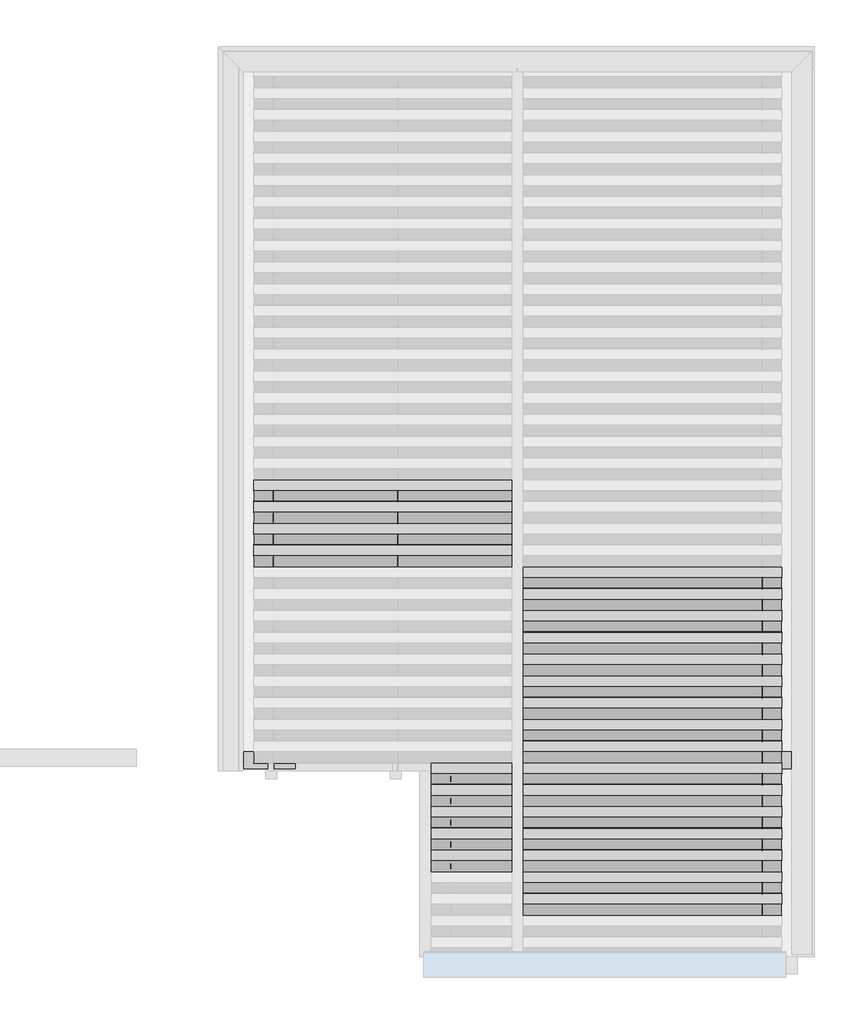
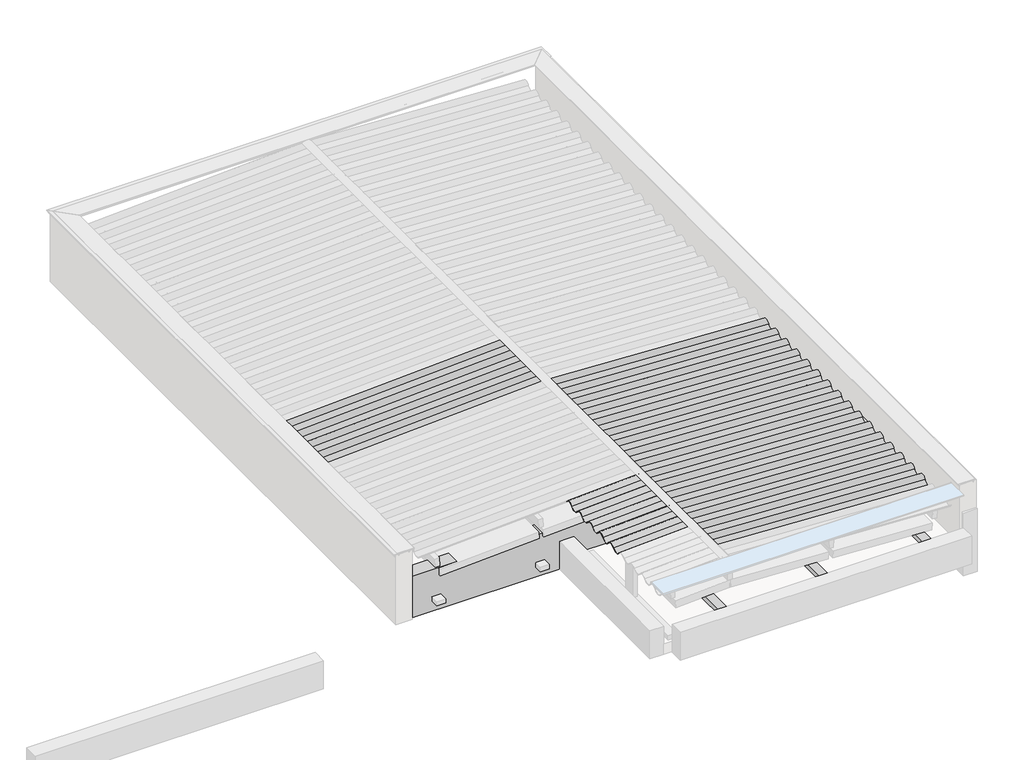
# One storey, part 2 of 4: 34 beams, 7 columns.
"""IFC4 building model written with IfcOpenShell, lengths in millimetres."""

import ifcopenshell
import ifcopenshell.guid

model = None  # the IFC model being written
_history = None  # IfcOwnerHistory: only IFC2X3 demands one
_inside = {}  # id of a spatial element -> (the spatial element, [elements in it])
_under = {}  # id of a project, library or spatial element -> (it, [spatial elements below it])
_declared = {}  # id of a project -> (the project, [libraries it declares])
_typed = {}  # id of a type object -> (the type object, [elements of that type])
_made_of = {}  # id of a material, layer set ... -> (it, [elements and type objects made of it])


def new_model(schema):
    """Start an empty IFC model of exactly this schema.

    Asked for "IFC4X3", IfcOpenShell would pick the latest addendum, in which some entities
    have other attributes; the version numbers below select the first issue.
    IFC2X3 requires an IfcOwnerHistory on every rooted entity: one is made here for all.
    """
    global model, _history
    if schema == "IFC4X3":
        model = ifcopenshell.file(schema_version=(4, 3, 0, 0))
    else:
        model = ifcopenshell.file(schema=schema)
    _inside.clear()
    _under.clear()
    _declared.clear()
    _typed.clear()
    _made_of.clear()
    _history = None
    if model.schema == "IFC2X3":
        org = make("IfcOrganization", Name="unknown")
        user = make(
            "IfcPersonAndOrganization",
            ThePerson=make("IfcPerson", FamilyName="unknown"),
            TheOrganization=org,
        )
        app = make(
            "IfcApplication",
            ApplicationDeveloper=org,
            Version="unknown",
            ApplicationFullName="unknown",
            ApplicationIdentifier="unknown",
        )
        _history = make(
            "IfcOwnerHistory",
            OwningUser=user,
            OwningApplication=app,
            ChangeAction="ADDED",
            CreationDate=0,
        )
    return model


def make(cls, **values):
    """One entity of the class cls with the attributes given. An attribute that is None is left unset."""
    return model.create_entity(
        cls, **{name: value for name, value in values.items() if value is not None}
    )


def rooted(cls, **values):
    """An entity with a GlobalId (a new one), such as an element, a storey or a relation."""
    return make(cls, GlobalId=ifcopenshell.guid.new(), OwnerHistory=_history, **values)


def si_unit(unit_type, name, prefix=None):
    """IfcSIUnit, for example si_unit("LENGTHUNIT", "METRE", prefix="MILLI")."""
    return make("IfcSIUnit", UnitType=unit_type, Prefix=prefix, Name=name)


def assignment(units):
    """IfcUnitAssignment: the units of a project."""
    return None if units is None else make("IfcUnitAssignment", Units=units)


def point(xyz):
    """IfcCartesianPoint."""
    return None if xyz is None else make("IfcCartesianPoint", Coordinates=xyz)


def direction(xyz):
    """IfcDirection."""
    return None if xyz is None else make("IfcDirection", DirectionRatios=xyz)


def frame(location, z_axis=None, x_axis=None):
    """IfcAxis2Placement3D, a coordinate frame: its origin and axes. An axis left out is left unset."""
    return make(
        "IfcAxis2Placement3D",
        Location=point(location),
        Axis=direction(z_axis),
        RefDirection=direction(x_axis),
    )


def frame_2d(location, x_axis=None):
    """IfcAxis2Placement2D, a coordinate frame in the plane: its origin and x axis."""
    return make(
        "IfcAxis2Placement2D", Location=point(location), RefDirection=direction(x_axis)
    )


def origin():
    """The frame at (0, 0, 0) with its axes left unset."""
    return frame((0.0, 0.0, 0.0))


def place(relative_to, where):
    """IfcLocalPlacement: puts the frame where relative to a parent placement (None: the world)."""
    return make(
        "IfcLocalPlacement", PlacementRelTo=relative_to, RelativePlacement=where
    )


def context(
    kind, dimensions, precision=None, world=None, true_north=None, identifier=None
):
    """IfcGeometricRepresentationContext, for example the 3D "Model" context."""
    return make(
        "IfcGeometricRepresentationContext",
        ContextIdentifier=identifier,
        ContextType=kind,
        CoordinateSpaceDimension=dimensions,
        Precision=precision,
        WorldCoordinateSystem=world,
        TrueNorth=true_north,
    )


def project(units=None, contexts=None):
    """IfcProject with its units and contexts."""
    return rooted(
        "IfcProject",
        Name="project",
        RepresentationContexts=contexts,
        UnitsInContext=assignment(units),
    )


def spatial(cls, under=None, at=None, **own):
    """A site, building, storey or space (cls), placed at a placement, below another one or the project."""
    s = rooted(cls, ObjectPlacement=at, **own)
    if under is not None:
        _under.setdefault(under.id(), (under, []))[1].append(s)
    return s


def polyline(points):
    """IfcPolyline through the points."""
    return make("IfcPolyline", Points=[point(p) for p in points])


def circle_curve(where, radius):
    """IfcCircle in the frame where."""
    return make("IfcCircle", Position=where, Radius=radius)


def trimmed(basis, trim1, trim2, sense, master):
    """IfcTrimmedCurve: the piece of a basis curve between two trims."""
    return make(
        "IfcTrimmedCurve",
        BasisCurve=basis,
        Trim1=trim1,
        Trim2=trim2,
        SenseAgreement=sense,
        MasterRepresentation=master,
    )


def segment(curve, same_sense, transition):
    """IfcCompositeCurveSegment."""
    return make(
        "IfcCompositeCurveSegment",
        Transition=transition,
        SameSense=same_sense,
        ParentCurve=curve,
    )


def composite_curve(segments, self_intersect=None):
    """IfcCompositeCurve: segments joined end to end."""
    return make("IfcCompositeCurve", Segments=segments, SelfIntersect=self_intersect)


def outline(outer, holes=None, kind="AREA"):
    """IfcArbitraryClosedProfileDef: a profile drawn as a closed curve; with holes, ...WithVoids."""
    if holes is None:
        return make("IfcArbitraryClosedProfileDef", ProfileType=kind, OuterCurve=outer)
    return make(
        "IfcArbitraryProfileDefWithVoids",
        ProfileType=kind,
        OuterCurve=outer,
        InnerCurves=holes,
    )


def extrude(swept, where, along, depth):
    """IfcExtrudedAreaSolid: the profile swept, set in the frame where, extruded along a direction by depth."""
    return make(
        "IfcExtrudedAreaSolid",
        SweptArea=swept,
        Position=where,
        ExtrudedDirection=direction(along),
        Depth=depth,
    )


def faces_of(points, faces, orient=None, outer=None):
    """IfcFace entities. A face is a list of loops; a loop is a list of indices into points, from 0.

    orient and outer hold one flag for each loop. By default every Orientation is true, the
    first loop of a face is its IfcFaceOuterBound and the others are IfcFaceBound.
    """
    made = []
    for i, loops in enumerate(faces):
        bounds = []
        for j, loop in enumerate(loops):
            is_outer = j == 0 if outer is None else outer[i][j]
            bounds.append(
                make(
                    "IfcFaceOuterBound" if is_outer else "IfcFaceBound",
                    Bound=make("IfcPolyLoop", Polygon=[points[k] for k in loop]),
                    Orientation=True if orient is None else orient[i][j],
                )
            )
        made.append(make("IfcFace", Bounds=bounds))
    return made


def faceted_brep(points, faces, orient=None, outer=None, voids=None):
    """IfcFacetedBrep: a solid bounded by flat faces; with voids (closed shells), ...WithVoids."""
    shared = [point(p) for p in points]
    hull = make("IfcClosedShell", CfsFaces=faces_of(shared, faces, orient, outer))
    if voids is None:
        return make("IfcFacetedBrep", Outer=hull)
    return make(
        "IfcFacetedBrepWithVoids",
        Outer=hull,
        Voids=[
            make(cls, CfsFaces=faces_of(shared, fs, o, b)) for cls, fs, o, b in voids
        ],
    )


def shape(context_of_items, identifier, shape_type, items):
    """IfcShapeRepresentation: the items that make up one representation, for example the "Body"."""
    return make(
        "IfcShapeRepresentation",
        ContextOfItems=context_of_items,
        RepresentationIdentifier=identifier,
        RepresentationType=shape_type,
        Items=items,
    )


def source(mapping_origin, context_of_items, identifier, shape_type, items):
    """IfcRepresentationMap: a shape defined once, which mapped items show again and again."""
    return make(
        "IfcRepresentationMap",
        MappingOrigin=mapping_origin,
        MappedRepresentation=shape(context_of_items, identifier, shape_type, items),
    )


def transform(
    local_origin,
    x_axis=None,
    y_axis=None,
    z_axis=None,
    scale=None,
    scale2=None,
    scale3=None,
    uniform=True,
):
    """IfcCartesianTransformationOperator3D, or its non-uniform kind. x_axis, y_axis, z_axis: its Axis1, 2, 3."""
    if uniform:
        return make(
            "IfcCartesianTransformationOperator3D",
            Axis1=direction(x_axis),
            Axis2=direction(y_axis),
            LocalOrigin=point(local_origin),
            Scale=scale,
            Axis3=direction(z_axis),
        )
    return make(
        "IfcCartesianTransformationOperator3DnonUniform",
        Axis1=direction(x_axis),
        Axis2=direction(y_axis),
        LocalOrigin=point(local_origin),
        Scale=scale,
        Axis3=direction(z_axis),
        Scale2=scale2,
        Scale3=scale3,
    )


def mapped(mapping_source, mapping_target):
    """IfcMappedItem: shows the shape of a source again, moved by a transform."""
    return make(
        "IfcMappedItem", MappingSource=mapping_source, MappingTarget=mapping_target
    )


def made_of(thing, what):
    """Note that an element or type object is made of a material, layer set ...; save() writes the relation."""
    if what is not None:
        _made_of.setdefault(what.id(), (what, []))[1].append(thing)
    return thing


def element(
    cls,
    number,
    at=None,
    inside=None,
    cuts=None,
    type_object=None,
    material=None,
    context=None,
    identifier="Body",
    shape_type=None,
    held_by="IfcProductDefinitionShape",
    body=None,
    shapes=None,
    **own,
):
    """One element of the class cls, such as IfcWall. Its Tag is "e" and its number.

    at: its placement. inside: the storey or other place that contains it. cuts: it is an
    opening in that element (IfcRelVoidsElement). A single representation is given by context,
    identifier, shape_type and body (its items); several are given by shapes. held_by: the class
    of the entity that holds the representations. save() writes the other relations.
    """
    e = rooted(cls, Tag="e%d" % number, ObjectPlacement=at, **own)
    if body is not None:
        shapes = [shape(context, identifier, shape_type, body)]
    if shapes is not None:
        e.Representation = make(held_by, Representations=shapes)
    if inside is not None:
        _inside.setdefault(inside.id(), (inside, []))[1].append(e)
    if cuts is not None:
        rooted(
            "IfcRelVoidsElement", RelatingBuildingElement=cuts, RelatedOpeningElement=e
        )
    if type_object is not None:
        _typed.setdefault(type_object.id(), (type_object, []))[1].append(e)
    return made_of(e, material)


def aggregate(whole, parts):
    """IfcRelAggregates: a whole, such as a stair, and the parts it consists of."""
    return rooted("IfcRelAggregates", RelatingObject=whole, RelatedObjects=parts)


def save(model, path):
    """Write the relations noted so far, then the file.

    IfcRelAggregates (storeys below a building ...), IfcRelContainedInSpatialStructure (elements
    in a storey), IfcRelDefinesByType, IfcRelAssociatesMaterial and IfcRelDeclares: one each for
    every whole, place, type object, material and project.
    """
    for whole, parts in _under.values():
        aggregate(whole, parts)
    for where, things in _inside.values():
        rooted(
            "IfcRelContainedInSpatialStructure",
            RelatedElements=things,
            RelatingStructure=where,
        )
    for kind, things in _typed.values():
        rooted("IfcRelDefinesByType", RelatedObjects=things, RelatingType=kind)
    for what, things in _made_of.values():
        rooted("IfcRelAssociatesMaterial", RelatedObjects=things, RelatingMaterial=what)
    for by, libraries in _declared.values():
        rooted("IfcRelDeclares", RelatingContext=by, RelatedDefinitions=libraries)
    model.write(path)


def column_f3930958(model_context):
    return source(origin(), model_context, "Body", "SweptSolid", [
        extrude(outline(polyline([(30.0, 80.0), (30.0, -80.0), (-30.0, -80.0), (-30.0, 80.0), (30.0, 80.0)])), frame((0.0, 0.0, 4460.0), z_axis=(0.0, 0.0, 1.0), x_axis=(1.0, 0.0, 0.0)), (0.0, 0.0, 1.0), 522.9),
    ])


def column_4d3918cc(model_context):
    return source(origin(), model_context, "Body", "SweptSolid", [
        extrude(outline(polyline([(30.0, 80.0), (30.0, -80.0), (-30.0, -80.0), (-30.0, 80.0), (30.0, 80.0)])), frame((0.0, 0.0, 4460.0), z_axis=(0.0, 0.0, 1.0), x_axis=(1.0, 0.0, 0.0)), (0.0, 0.0, 1.0), 426.9),
    ])


def column_924cc83b(model_context):
    return source(origin(), model_context, "Body", "SweptSolid", [
        extrude(outline(polyline([(30.0, 80.0), (30.0, -80.0), (-30.0, -80.0), (-30.0, 80.0), (30.0, 80.0)])), frame((0.0, 0.0, 4460.0), z_axis=(0.0, 0.0, 1.0), x_axis=(1.0, 0.0, 0.0)), (0.0, 0.0, 1.0), 497.0),
    ])


model = new_model("IFC4")

# Units and contexts
model_context = context("Model", 3, world=origin())
ifc_project = project(units=[si_unit("LENGTHUNIT", "METRE", prefix="MILLI")], contexts=[model_context])

# Site, building, storey
site = spatial("IfcSite", under=ifc_project)
building = spatial("IfcBuilding", under=site)
storey = spatial("IfcBuildingStorey", under=building, Name="COB. SALA ESTAR", Elevation=4400.0)

# Beams
placement = place(None, origin())
element("IfcBeam", 1, ObjectType="Madeira de lei : Berço 6x12cm", at=placement, inside=storey, context=model_context, shape_type="SweptSolid", body=[
    extrude(outline(polyline([(-3400.781307, -376.0699847), (-3280.781307, -376.0699847), (-3280.781307, -2376.0699847), (-3400.781307, -2376.0699847), (-3400.781307, -376.0699847)])), frame((0.0, 0.0, 4400.0), z_axis=(0.0, 0.0, 1.0), x_axis=(1.0, 0.0, 0.0)), (0.0, 0.0, 1.0), 60.0),
])
element("IfcBeam", 2, ObjectType="Madeira de lei : Berço 6x12cm", at=placement, inside=storey, context=model_context, shape_type="SweptSolid", body=[
    extrude(outline(polyline([(-3400.781307, -2376.0699847), (-3280.781307, -2376.0699847), (-3280.781307, -4336.0699847), (-3400.781307, -4336.0699847), (-3400.781307, -2376.0699847)])), frame((0.0, 0.0, 4400.0), z_axis=(0.0, 0.0, 1.0), x_axis=(1.0, 0.0, 0.0)), (0.0, 0.0, 1.0), 60.0),
])
element("IfcBeam", 3, ObjectType="Madeira de lei : Berço 6x12cm", at=placement, inside=storey, context=model_context, shape_type="SweptSolid", body=[
    extrude(outline(polyline([(-2032.4438771, -376.0699847), (-1912.4438771, -376.0699847), (-1912.4438771, -2376.0699847), (-2032.4438771, -2376.0699847), (-2032.4438771, -376.0699847)])), frame((0.0, 0.0, 4400.0), z_axis=(0.0, 0.0, 1.0), x_axis=(1.0, 0.0, 0.0)), (0.0, 0.0, 1.0), 60.0),
])
element("IfcBeam", 4, ObjectType="Madeira de lei : Berço 6x12cm", at=placement, inside=storey, context=model_context, shape_type="SweptSolid", body=[
    extrude(outline(polyline([(-2032.4438771, -2376.0699847), (-1912.4438771, -2376.0699847), (-1912.4438771, -4336.0699847), (-2032.4438771, -4336.0699847), (-2032.4438771, -2376.0699847)])), frame((0.0, 0.0, 4400.0), z_axis=(0.0, 0.0, 1.0), x_axis=(1.0, 0.0, 0.0)), (0.0, 0.0, 1.0), 60.0),
])
element("IfcBeam", 5, ObjectType="Madeira de lei : Berço 6x12cm", at=placement, inside=storey, context=model_context, shape_type="SweptSolid", body=[
    extrude(outline(polyline([(-634.1438771, -376.0699847), (-514.1438771, -376.0699847), (-514.1438771, -2376.0699847), (-634.1438771, -2376.0699847), (-634.1438771, -376.0699847)])), frame((0.0, 0.0, 4400.0), z_axis=(0.0, 0.0, 1.0), x_axis=(1.0, 0.0, 0.0)), (0.0, 0.0, 1.0), 60.0),
])
element("IfcBeam", 6, ObjectType="Madeira de lei : Berço 6x12cm", at=placement, inside=storey, context=model_context, shape_type="SweptSolid", body=[
    extrude(outline(polyline([(-634.1438771, -2376.0699847), (-514.1438771, -2376.0699847), (-514.1438771, -4336.0699847), (-634.1438771, -4336.0699847), (-634.1438771, -2376.0699847)])), frame((0.0, 0.0, 4400.0), z_axis=(0.0, 0.0, 1.0), x_axis=(1.0, 0.0, 0.0)), (0.0, 0.0, 1.0), 60.0),
])
element("IfcBeam", 7, ObjectType="Madeira de lei : Berço 6x12cm", at=placement, inside=storey, context=model_context, shape_type="SweptSolid", body=[
    extrude(outline(polyline([(-6167.4187368, 1623.9300153), (-6047.4187368, 1623.9300153), (-6047.4187368, -376.0699847), (-6167.4187368, -376.0699847), (-6167.4187368, 1623.9300153)])), frame((0.0, 0.0, 4400.0), z_axis=(0.0, 0.0, 1.0), x_axis=(1.0, 0.0, 0.0)), (0.0, 0.0, 1.0), 60.0),
])
element("IfcBeam", 8, ObjectType="TQS - Viga retangular : 19.0 x 60.0", at=placement, inside=storey, context=model_context, shape_type="Brep", body=[
    faceted_brep([(-6630.281307, -174.5699847, 4850.0), (-6440.281307, -174.5699847, 4850.0), (-6440.281307, 5584.4300153, 4850.0), (-6630.281307, 5584.4300153, 4850.0), (-6440.281307, -174.5699847, 4250.0), (-6440.281307, 5584.4300153, 4250.0), (-6440.281307, 5584.4300153, 4400.0), (-6630.281307, -174.5699847, 4250.0), (-6630.281307, 5584.4300153, 4250.0)], [[[0, 1, 2, 3]], [[1, 4, 5, 6, 2]], [[4, 7, 8, 5]], [[7, 0, 3, 8]], [[1, 0, 7, 4]], [[3, 2, 6, 5, 8]]]),
    faceted_brep([(-6630.281307, -424.5699847, 4850.0), (-6440.281307, -424.5699847, 4850.0), (-6440.281307, -424.5699847, 4250.0), (-6630.281307, -424.5699847, 4250.0), (-6630.281307, -2044.5699847, 4850.0), (-6440.281307, -2044.5699847, 4850.0), (-6440.281307, -2044.5699847, 4250.0), (-6630.281307, -2044.5699847, 4250.0)], [[[0, 1, 2, 3]], [[1, 0, 4, 5]], [[2, 1, 5, 6]], [[3, 2, 6, 7]], [[0, 3, 7, 4]], [[5, 4, 7, 6]]]),
    faceted_brep([(-6440.281307, -2259.5699847, 4850.0), (-6630.281307, -2259.5699847, 4850.0), (-6630.281307, -2259.5699847, 4250.0), (-6440.281307, -2259.5699847, 4250.0), (-6630.281307, -2234.5699847, 4850.0), (-6440.281307, -2234.5699847, 4850.0), (-6440.281307, -2234.5699847, 4250.0), (-6630.281307, -2234.5699847, 4250.0)], [[[0, 1, 2, 3]], [[4, 5, 6, 7]], [[1, 0, 5, 4]], [[0, 3, 6, 5]], [[3, 2, 7, 6]], [[2, 1, 4, 7]]]),
])
element("IfcBeam", 9, ObjectType="TQS - Viga retangular : 19.0 x 60.0", at=placement, inside=storey, context=model_context, shape_type="Brep", body=[
    faceted_brep([(-202.6220088, -2259.5699847, 4850.0), (-202.6137562, -2069.5699847, 4850.0), (-6440.281307, -2069.5699847, 4850.0), (-6440.281307, -2234.5699847, 4850.0), (-6440.281307, -2259.5699847, 4850.0), (-202.6220088, -2259.5699847, 4250.0), (-202.6220088, -2259.5699847, 4400.0), (-6440.281307, -2259.5699847, 4250.0), (-4252.481307, -2259.5699847, 4250.0), (-202.6137562, -2069.5699847, 4250.0), (-6440.281307, -2234.5699847, 4250.0), (-6440.281307, -2069.5699847, 4250.0), (-202.6137562, -2069.5699847, 4400.0), (-6440.281307, -2069.5699847, 4400.0)], [[[0, 1, 2, 3, 4]], [[5, 6, 0, 4, 7, 8]], [[9, 5, 8, 7, 10, 11]], [[1, 12, 9, 11, 13, 2]], [[2, 13, 11, 10, 7, 4, 3]], [[1, 0, 6, 5, 9, 12]]]),
])
element("IfcBeam", 10, ObjectType="Telha Ondulada : Fibrocimento", at=placement, inside=storey, context=model_context, shape_type="SweptSolid", body=[
    extrude(outline(composite_curve([segment(trimmed(circle_curve(frame_2d((-58.7002978, -53.2060538)), 66.7939461), [point((-29.3501489, 6.7939462))], [point((-29.3501489, -113.2060538))], False, "CARTESIAN"), True, "CONTINUOUS"), segment(polyline([(-29.3501489, -113.2060538), (-31.5472154, -108.7146288)]), True, "CONTINUOUS"), segment(trimmed(circle_curve(frame_2d((-58.7002978, -53.2060538)), 61.7939461), [point((-31.5472154, -108.7146288))], [point((-31.5472154, 2.3025211))], True, "CARTESIAN"), True, "CONTINUOUS"), segment(trimmed(circle_curve(frame_2d((0.0, 66.7939462)), 71.7939461), [point((-31.5472154, 2.3025211))], [point((-31.5472154, 131.2853712))], False, "CARTESIAN"), True, "CONTINUOUS"), segment(polyline([(-31.5472154, 131.2853712), (-29.3501489, 126.7939462)]), True, "CONTINUOUS"), segment(trimmed(circle_curve(frame_2d((0.0, 66.7939462)), 66.7939461), [point((-29.3501489, 126.7939462))], [point((-29.3501489, 6.7939462))], True, "CARTESIAN"), True, "CONTINUOUS")], self_intersect=False)), frame((-4311.894473, -3289.673052, 5167.7128806), z_axis=(0.9987523388778448, 0.0, 0.049937616943891816), x_axis=(-0.049937616943891816, 0.0, 0.9987523388778448)), (0.0, 0.0, 1.0), 967.7366024),
])
element("IfcBeam", 11, ObjectType="Telha Ondulada : Fibrocimento", at=placement, inside=storey, context=model_context, shape_type="SweptSolid", body=[
    extrude(outline(composite_curve([segment(trimmed(circle_curve(frame_2d((-58.7002978, -53.2060538)), 66.7939461), [point((-29.3501489, 6.7939462))], [point((-29.3501489, -113.2060538))], False, "CARTESIAN"), True, "CONTINUOUS"), segment(polyline([(-29.3501489, -113.2060538), (-31.5472154, -108.7146288)]), True, "CONTINUOUS"), segment(trimmed(circle_curve(frame_2d((-58.7002978, -53.2060538)), 61.7939461), [point((-31.5472154, -108.7146288))], [point((-31.5472154, 2.3025211))], True, "CARTESIAN"), True, "CONTINUOUS"), segment(trimmed(circle_curve(frame_2d((0.0, 66.7939462)), 71.7939461), [point((-31.5472154, 2.3025211))], [point((-31.5472154, 131.2853712))], False, "CARTESIAN"), True, "CONTINUOUS"), segment(polyline([(-31.5472154, 131.2853712), (-29.3501489, 126.7939462)]), True, "CONTINUOUS"), segment(trimmed(circle_curve(frame_2d((0.0, 66.7939462)), 66.7939461), [point((-29.3501489, 126.7939462))], [point((-29.3501489, 6.7939462))], True, "CARTESIAN"), True, "CONTINUOUS")], self_intersect=False)), frame((-4311.894473, -3045.173052, 5167.7128806), z_axis=(0.9987523388778448, 0.0, 0.049937616943891816), x_axis=(-0.049937616943891816, 0.0, 0.9987523388778448)), (0.0, 0.0, 1.0), 967.7366024),
])
element("IfcBeam", 12, ObjectType="Telha Ondulada : Fibrocimento", at=placement, inside=storey, context=model_context, shape_type="SweptSolid", body=[
    extrude(outline(composite_curve([segment(trimmed(circle_curve(frame_2d((-58.7002978, -53.2060538)), 66.7939461), [point((-29.3501489, 6.7939462))], [point((-29.3501489, -113.2060538))], False, "CARTESIAN"), True, "CONTINUOUS"), segment(polyline([(-29.3501489, -113.2060538), (-31.5472154, -108.7146288)]), True, "CONTINUOUS"), segment(trimmed(circle_curve(frame_2d((-58.7002978, -53.2060538)), 61.7939461), [point((-31.5472154, -108.7146288))], [point((-31.5472154, 2.3025211))], True, "CARTESIAN"), True, "CONTINUOUS"), segment(trimmed(circle_curve(frame_2d((0.0, 66.7939462)), 71.7939461), [point((-31.5472154, 2.3025211))], [point((-31.5472154, 131.2853712))], False, "CARTESIAN"), True, "CONTINUOUS"), segment(polyline([(-31.5472154, 131.2853712), (-29.3501489, 126.7939462)]), True, "CONTINUOUS"), segment(trimmed(circle_curve(frame_2d((0.0, 66.7939462)), 66.7939461), [point((-29.3501489, 126.7939462))], [point((-29.3501489, 6.7939462))], True, "CARTESIAN"), True, "CONTINUOUS")], self_intersect=False)), frame((-4311.894473, -2800.673052, 5167.7128806), z_axis=(0.9987523388778448, 0.0, 0.049937616943891844), x_axis=(-0.049937616943891844, 0.0, 0.9987523388778448)), (0.0, 0.0, 1.0), 967.7366024),
])
element("IfcBeam", 13, ObjectType="Telha Ondulada : Fibrocimento", at=placement, inside=storey, context=model_context, shape_type="SweptSolid", body=[
    extrude(outline(composite_curve([segment(trimmed(circle_curve(frame_2d((-58.7002978, -53.2060538)), 66.7939461), [point((-29.3501489, 6.7939462))], [point((-29.3501489, -113.2060538))], False, "CARTESIAN"), True, "CONTINUOUS"), segment(polyline([(-29.3501489, -113.2060538), (-31.5472154, -108.7146288)]), True, "CONTINUOUS"), segment(trimmed(circle_curve(frame_2d((-58.7002978, -53.2060538)), 61.7939461), [point((-31.5472154, -108.7146288))], [point((-31.5472154, 2.3025211))], True, "CARTESIAN"), True, "CONTINUOUS"), segment(trimmed(circle_curve(frame_2d((0.0, 66.7939462)), 71.7939461), [point((-31.5472154, 2.3025211))], [point((-31.5472154, 131.2853712))], False, "CARTESIAN"), True, "CONTINUOUS"), segment(polyline([(-31.5472154, 131.2853712), (-29.3501489, 126.7939462)]), True, "CONTINUOUS"), segment(trimmed(circle_curve(frame_2d((0.0, 66.7939462)), 66.7939461), [point((-29.3501489, 126.7939462))], [point((-29.3501489, 6.7939462))], True, "CARTESIAN"), True, "CONTINUOUS")], self_intersect=False)), frame((-4311.894473, -2556.173052, 5167.7128806), z_axis=(0.9987523388778448, 0.0, 0.049937616943891816), x_axis=(-0.049937616943891816, 0.0, 0.9987523388778448)), (0.0, 0.0, 1.0), 967.7366024),
])
element("IfcBeam", 14, ObjectType="Telha Ondulada : Fibrocimento", at=placement, inside=storey, context=model_context, shape_type="SweptSolid", body=[
    extrude(outline(composite_curve([segment(trimmed(circle_curve(frame_2d((-58.7002978, -53.2060538)), 66.7939461), [point((-29.3501489, 6.7939462))], [point((-29.3501489, -113.2060538))], False, "CARTESIAN"), True, "CONTINUOUS"), segment(polyline([(-29.3501489, -113.2060538), (-31.5472154, -108.7146288)]), True, "CONTINUOUS"), segment(trimmed(circle_curve(frame_2d((-58.7002978, -53.2060538)), 61.7939461), [point((-31.5472154, -108.7146288))], [point((-31.5472154, 2.3025211))], True, "CARTESIAN"), True, "CONTINUOUS"), segment(trimmed(circle_curve(frame_2d((0.0, 66.7939462)), 71.7939461), [point((-31.5472154, 2.3025211))], [point((-31.5472154, 131.2853712))], False, "CARTESIAN"), True, "CONTINUOUS"), segment(polyline([(-31.5472154, 131.2853712), (-29.3501489, 126.7939462)]), True, "CONTINUOUS"), segment(trimmed(circle_curve(frame_2d((0.0, 66.7939462)), 66.7939461), [point((-29.3501489, 126.7939462))], [point((-29.3501489, 6.7939462))], True, "CARTESIAN"), True, "CONTINUOUS")], self_intersect=False)), frame((-4311.894473, -2311.673052, 5167.7128806), z_axis=(0.9987523388778448, 0.0, 0.04993761694389179), x_axis=(-0.04993761694389179, 0.0, 0.9987523388778448)), (0.0, 0.0, 1.0), 967.7366024),
])
element("IfcBeam", 15, ObjectType="Telha Ondulada : Fibrocimento", at=placement, inside=storey, context=model_context, shape_type="SweptSolid", body=[
    extrude(outline(composite_curve([segment(trimmed(circle_curve(frame_2d((-58.7002978, -53.2060538)), 66.7939461), [point((-29.3501488, 6.7939462))], [point((-29.3501488, -113.2060538))], False, "CARTESIAN"), True, "CONTINUOUS"), segment(polyline([(-29.3501488, -113.2060538), (-31.5472154, -108.7146288)]), True, "CONTINUOUS"), segment(trimmed(circle_curve(frame_2d((-58.7002978, -53.2060538)), 61.7939461), [point((-31.5472154, -108.7146288))], [point((-31.5472154, 2.3025211))], True, "CARTESIAN"), True, "CONTINUOUS"), segment(trimmed(circle_curve(frame_2d((0.0, 66.7939462)), 71.7939461), [point((-31.5472154, 2.3025211))], [point((-31.5472154, 131.2853712))], False, "CARTESIAN"), True, "CONTINUOUS"), segment(polyline([(-31.5472154, 131.2853712), (-29.3501488, 126.7939462)]), True, "CONTINUOUS"), segment(trimmed(circle_curve(frame_2d((0.0, 66.7939462)), 66.7939461), [point((-29.3501488, 126.7939462))], [point((-29.3501488, 6.7939462))], True, "CARTESIAN"), True, "CONTINUOUS")], self_intersect=False)), frame((-6303.6781287, 133.326948, 5068.1236978), z_axis=(0.9987523388778448, 0.0, 0.049937616943891344), x_axis=(-0.049937616943891344, 0.0, 0.9987523388778448)), (0.0, 0.0, 1.0), 2962.0084336),
])
element("IfcBeam", 16, ObjectType="Telha Ondulada : Fibrocimento", at=placement, inside=storey, context=model_context, shape_type="SweptSolid", body=[
    extrude(outline(composite_curve([segment(trimmed(circle_curve(frame_2d((-58.7002978, -53.2060538)), 66.7939461), [point((-29.3501488, 6.7939462))], [point((-29.3501488, -113.2060538))], False, "CARTESIAN"), True, "CONTINUOUS"), segment(polyline([(-29.3501488, -113.2060538), (-31.5472154, -108.7146288)]), True, "CONTINUOUS"), segment(trimmed(circle_curve(frame_2d((-58.7002978, -53.2060538)), 61.7939461), [point((-31.5472154, -108.7146288))], [point((-31.5472154, 2.3025211))], True, "CARTESIAN"), True, "CONTINUOUS"), segment(trimmed(circle_curve(frame_2d((0.0, 66.7939462)), 71.7939461), [point((-31.5472154, 2.3025211))], [point((-31.5472154, 131.2853712))], False, "CARTESIAN"), True, "CONTINUOUS"), segment(polyline([(-31.5472154, 131.2853712), (-29.3501488, 126.7939462)]), True, "CONTINUOUS"), segment(trimmed(circle_curve(frame_2d((0.0, 66.7939462)), 66.7939461), [point((-29.3501488, 126.7939462))], [point((-29.3501488, 6.7939462))], True, "CARTESIAN"), True, "CONTINUOUS")], self_intersect=False)), frame((-6303.6781287, 377.826948, 5068.1236978), z_axis=(0.9987523388778449, 0.0, 0.049937616943891365), x_axis=(-0.049937616943891365, 0.0, 0.9987523388778449)), (0.0, 0.0, 1.0), 2962.0084336),
])
element("IfcBeam", 17, ObjectType="Telha Ondulada : Fibrocimento", at=placement, inside=storey, context=model_context, shape_type="SweptSolid", body=[
    extrude(outline(composite_curve([segment(trimmed(circle_curve(frame_2d((-58.7002978, -53.2060538)), 66.7939461), [point((-29.3501488, 6.7939462))], [point((-29.3501488, -113.2060538))], False, "CARTESIAN"), True, "CONTINUOUS"), segment(polyline([(-29.3501488, -113.2060538), (-31.5472154, -108.7146288)]), True, "CONTINUOUS"), segment(trimmed(circle_curve(frame_2d((-58.7002978, -53.2060538)), 61.7939461), [point((-31.5472154, -108.7146288))], [point((-31.5472154, 2.3025211))], True, "CARTESIAN"), True, "CONTINUOUS"), segment(trimmed(circle_curve(frame_2d((0.0, 66.7939462)), 71.7939461), [point((-31.5472154, 2.3025211))], [point((-31.5472154, 131.2853712))], False, "CARTESIAN"), True, "CONTINUOUS"), segment(polyline([(-31.5472154, 131.2853712), (-29.3501488, 126.7939462)]), True, "CONTINUOUS"), segment(trimmed(circle_curve(frame_2d((0.0, 66.7939462)), 66.7939461), [point((-29.3501488, 126.7939462))], [point((-29.3501488, 6.7939462))], True, "CARTESIAN"), True, "CONTINUOUS")], self_intersect=False)), frame((-6303.6781287, 622.326948, 5068.1236978), z_axis=(0.9987523388778448, 0.0, 0.04993761694389136), x_axis=(-0.04993761694389136, 0.0, 0.9987523388778448)), (0.0, 0.0, 1.0), 2962.0084336),
])
element("IfcBeam", 18, ObjectType="Telha Ondulada : Fibrocimento", at=placement, inside=storey, context=model_context, shape_type="SweptSolid", body=[
    extrude(outline(composite_curve([segment(trimmed(circle_curve(frame_2d((-58.7002978, -53.2060538)), 66.7939461), [point((-29.3501488, 6.7939462))], [point((-29.3501488, -113.2060538))], False, "CARTESIAN"), True, "CONTINUOUS"), segment(polyline([(-29.3501488, -113.2060538), (-31.5472154, -108.7146288)]), True, "CONTINUOUS"), segment(trimmed(circle_curve(frame_2d((-58.7002978, -53.2060538)), 61.7939461), [point((-31.5472154, -108.7146288))], [point((-31.5472154, 2.3025211))], True, "CARTESIAN"), True, "CONTINUOUS"), segment(trimmed(circle_curve(frame_2d((0.0, 66.7939462)), 71.7939461), [point((-31.5472154, 2.3025211))], [point((-31.5472154, 131.2853712))], False, "CARTESIAN"), True, "CONTINUOUS"), segment(polyline([(-31.5472154, 131.2853712), (-29.3501488, 126.7939462)]), True, "CONTINUOUS"), segment(trimmed(circle_curve(frame_2d((0.0, 66.7939462)), 66.7939461), [point((-29.3501488, 126.7939462))], [point((-29.3501488, 6.7939462))], True, "CARTESIAN"), True, "CONTINUOUS")], self_intersect=False)), frame((-6303.6781287, 866.826948, 5068.1236978), z_axis=(0.9987523388778448, 0.0, 0.04993761694389134), x_axis=(-0.04993761694389134, 0.0, 0.9987523388778448)), (0.0, 0.0, 1.0), 2962.0084336),
])
element("IfcBeam", 19, ObjectType="Telha Ondulada : Fibrocimento", at=placement, inside=storey, context=model_context, shape_type="SweptSolid", body=[
    extrude(outline(composite_curve([segment(trimmed(circle_curve(frame_2d((0.0, 66.7939462)), 66.7939461), [point((29.3501488, 6.7939462))], [point((29.3501488, 126.7939462))], True, "CARTESIAN"), True, "CONTINUOUS"), segment(polyline([(29.3501488, 126.7939462), (31.5472154, 131.2853712)]), True, "CONTINUOUS"), segment(trimmed(circle_curve(frame_2d((0.0, 66.7939462)), 71.7939461), [point((31.5472154, 131.2853712))], [point((31.5472154, 2.3025211))], False, "CARTESIAN"), True, "CONTINUOUS"), segment(trimmed(circle_curve(frame_2d((58.7002978, -53.2060538)), 61.7939461), [point((31.5472154, 2.3025211))], [point((31.5472154, -108.7146288))], True, "CARTESIAN"), True, "CONTINUOUS"), segment(polyline([(31.5472154, -108.7146288), (29.3501488, -113.2060538)]), True, "CONTINUOUS"), segment(trimmed(circle_curve(frame_2d((58.7002978, -53.2060538)), 66.7939461), [point((29.3501488, -113.2060538))], [point((29.3501488, 6.7939462))], False, "CARTESIAN"), True, "CONTINUOUS")], self_intersect=False)), frame((-377.8844852, -3778.673052, 5068.1236978), z_axis=(-0.9987523388778448, 0.0, 0.049937616943891455), x_axis=(-0.049937616943891455, 0.0, -0.9987523388778448)), (0.0, 0.0, 1.0), 2962.0084336),
])
element("IfcBeam", 20, ObjectType="Telha Ondulada : Fibrocimento", at=placement, inside=storey, context=model_context, shape_type="SweptSolid", body=[
    extrude(outline(composite_curve([segment(trimmed(circle_curve(frame_2d((0.0, 66.7939462)), 66.7939461), [point((29.3501488, 6.7939462))], [point((29.3501488, 126.7939462))], True, "CARTESIAN"), True, "CONTINUOUS"), segment(polyline([(29.3501488, 126.7939462), (31.5472154, 131.2853712)]), True, "CONTINUOUS"), segment(trimmed(circle_curve(frame_2d((0.0, 66.7939462)), 71.7939461), [point((31.5472154, 131.2853712))], [point((31.5472154, 2.3025211))], False, "CARTESIAN"), True, "CONTINUOUS"), segment(trimmed(circle_curve(frame_2d((58.7002978, -53.2060538)), 61.7939461), [point((31.5472154, 2.3025211))], [point((31.5472154, -108.7146288))], True, "CARTESIAN"), True, "CONTINUOUS"), segment(polyline([(31.5472154, -108.7146288), (29.3501488, -113.2060538)]), True, "CONTINUOUS"), segment(trimmed(circle_curve(frame_2d((58.7002978, -53.2060538)), 66.7939461), [point((29.3501488, -113.2060538))], [point((29.3501488, 6.7939462))], False, "CARTESIAN"), True, "CONTINUOUS")], self_intersect=False)), frame((-377.8844852, -3534.173052, 5068.1236978), z_axis=(-0.9987523388778448, 0.0, 0.049937616943891455), x_axis=(-0.049937616943891455, 0.0, -0.9987523388778448)), (0.0, 0.0, 1.0), 2962.0084336),
])
element("IfcBeam", 21, ObjectType="Telha Ondulada : Fibrocimento", at=placement, inside=storey, context=model_context, shape_type="SweptSolid", body=[
    extrude(outline(composite_curve([segment(trimmed(circle_curve(frame_2d((0.0, 66.7939462)), 66.7939461), [point((29.3501488, 6.7939462))], [point((29.3501488, 126.7939462))], True, "CARTESIAN"), True, "CONTINUOUS"), segment(polyline([(29.3501488, 126.7939462), (31.5472154, 131.2853712)]), True, "CONTINUOUS"), segment(trimmed(circle_curve(frame_2d((0.0, 66.7939462)), 71.7939461), [point((31.5472154, 131.2853712))], [point((31.5472154, 2.3025211))], False, "CARTESIAN"), True, "CONTINUOUS"), segment(trimmed(circle_curve(frame_2d((58.7002978, -53.2060538)), 61.7939461), [point((31.5472154, 2.3025211))], [point((31.5472154, -108.7146288))], True, "CARTESIAN"), True, "CONTINUOUS"), segment(polyline([(31.5472154, -108.7146288), (29.3501488, -113.2060538)]), True, "CONTINUOUS"), segment(trimmed(circle_curve(frame_2d((58.7002978, -53.2060538)), 66.7939461), [point((29.3501488, -113.2060538))], [point((29.3501488, 6.7939462))], False, "CARTESIAN"), True, "CONTINUOUS")], self_intersect=False)), frame((-377.8844852, -3289.673052, 5068.1236978), z_axis=(-0.9987523388778448, 0.0, 0.049937616943891455), x_axis=(-0.049937616943891455, 0.0, -0.9987523388778448)), (0.0, 0.0, 1.0), 2962.0084336),
])
element("IfcBeam", 22, ObjectType="Telha Ondulada : Fibrocimento", at=placement, inside=storey, context=model_context, shape_type="SweptSolid", body=[
    extrude(outline(composite_curve([segment(trimmed(circle_curve(frame_2d((0.0, 66.7939462)), 66.7939461), [point((29.3501488, 6.7939462))], [point((29.3501488, 126.7939462))], True, "CARTESIAN"), True, "CONTINUOUS"), segment(polyline([(29.3501488, 126.7939462), (31.5472154, 131.2853712)]), True, "CONTINUOUS"), segment(trimmed(circle_curve(frame_2d((0.0, 66.7939462)), 71.7939461), [point((31.5472154, 131.2853712))], [point((31.5472154, 2.3025211))], False, "CARTESIAN"), True, "CONTINUOUS"), segment(trimmed(circle_curve(frame_2d((58.7002978, -53.2060538)), 61.7939461), [point((31.5472154, 2.3025211))], [point((31.5472154, -108.7146288))], True, "CARTESIAN"), True, "CONTINUOUS"), segment(polyline([(31.5472154, -108.7146288), (29.3501488, -113.2060538)]), True, "CONTINUOUS"), segment(trimmed(circle_curve(frame_2d((58.7002978, -53.2060538)), 66.7939461), [point((29.3501488, -113.2060538))], [point((29.3501488, 6.7939462))], False, "CARTESIAN"), True, "CONTINUOUS")], self_intersect=False)), frame((-377.8844852, -3045.173052, 5068.1236978), z_axis=(-0.9987523388778448, 0.0, 0.049937616943891455), x_axis=(-0.049937616943891455, 0.0, -0.9987523388778448)), (0.0, 0.0, 1.0), 2962.0084336),
])
element("IfcBeam", 23, ObjectType="Telha Ondulada : Fibrocimento", at=placement, inside=storey, context=model_context, shape_type="SweptSolid", body=[
    extrude(outline(composite_curve([segment(trimmed(circle_curve(frame_2d((0.0, 66.7939462)), 66.7939461), [point((29.3501488, 6.7939462))], [point((29.3501488, 126.7939462))], True, "CARTESIAN"), True, "CONTINUOUS"), segment(polyline([(29.3501488, 126.7939462), (31.5472154, 131.2853712)]), True, "CONTINUOUS"), segment(trimmed(circle_curve(frame_2d((0.0, 66.7939462)), 71.7939461), [point((31.5472154, 131.2853712))], [point((31.5472154, 2.3025211))], False, "CARTESIAN"), True, "CONTINUOUS"), segment(trimmed(circle_curve(frame_2d((58.7002978, -53.2060538)), 61.7939461), [point((31.5472154, 2.3025211))], [point((31.5472154, -108.7146288))], True, "CARTESIAN"), True, "CONTINUOUS"), segment(polyline([(31.5472154, -108.7146288), (29.3501488, -113.2060538)]), True, "CONTINUOUS"), segment(trimmed(circle_curve(frame_2d((58.7002978, -53.2060538)), 66.7939461), [point((29.3501488, -113.2060538))], [point((29.3501488, 6.7939462))], False, "CARTESIAN"), True, "CONTINUOUS")], self_intersect=False)), frame((-377.8844852, -2800.673052, 5068.1236978), z_axis=(-0.9987523388778448, 0.0, 0.049937616943891455), x_axis=(-0.049937616943891455, 0.0, -0.9987523388778448)), (0.0, 0.0, 1.0), 2962.0084336),
])
element("IfcBeam", 24, ObjectType="Telha Ondulada : Fibrocimento", at=placement, inside=storey, context=model_context, shape_type="SweptSolid", body=[
    extrude(outline(composite_curve([segment(trimmed(circle_curve(frame_2d((0.0, 66.7939462)), 66.7939461), [point((29.3501488, 6.7939462))], [point((29.3501488, 126.7939462))], True, "CARTESIAN"), True, "CONTINUOUS"), segment(polyline([(29.3501488, 126.7939462), (31.5472154, 131.2853712)]), True, "CONTINUOUS"), segment(trimmed(circle_curve(frame_2d((0.0, 66.7939462)), 71.7939461), [point((31.5472154, 131.2853712))], [point((31.5472154, 2.3025211))], False, "CARTESIAN"), True, "CONTINUOUS"), segment(trimmed(circle_curve(frame_2d((58.7002978, -53.2060538)), 61.7939461), [point((31.5472154, 2.3025211))], [point((31.5472154, -108.7146288))], True, "CARTESIAN"), True, "CONTINUOUS"), segment(polyline([(31.5472154, -108.7146288), (29.3501488, -113.2060538)]), True, "CONTINUOUS"), segment(trimmed(circle_curve(frame_2d((58.7002978, -53.2060538)), 66.7939461), [point((29.3501488, -113.2060538))], [point((29.3501488, 6.7939462))], False, "CARTESIAN"), True, "CONTINUOUS")], self_intersect=False)), frame((-377.8844852, -2556.173052, 5068.1236978), z_axis=(-0.9987523388778448, 0.0, 0.049937616943891455), x_axis=(-0.049937616943891455, 0.0, -0.9987523388778448)), (0.0, 0.0, 1.0), 2962.0084336),
])
element("IfcBeam", 25, ObjectType="Telha Ondulada : Fibrocimento", at=placement, inside=storey, context=model_context, shape_type="SweptSolid", body=[
    extrude(outline(composite_curve([segment(trimmed(circle_curve(frame_2d((0.0, 66.7939462)), 66.7939461), [point((29.3501488, 6.7939462))], [point((29.3501488, 126.7939462))], True, "CARTESIAN"), True, "CONTINUOUS"), segment(polyline([(29.3501488, 126.7939462), (31.5472154, 131.2853712)]), True, "CONTINUOUS"), segment(trimmed(circle_curve(frame_2d((0.0, 66.7939462)), 71.7939461), [point((31.5472154, 131.2853712))], [point((31.5472154, 2.3025211))], False, "CARTESIAN"), True, "CONTINUOUS"), segment(trimmed(circle_curve(frame_2d((58.7002978, -53.2060538)), 61.7939461), [point((31.5472154, 2.3025211))], [point((31.5472154, -108.7146288))], True, "CARTESIAN"), True, "CONTINUOUS"), segment(polyline([(31.5472154, -108.7146288), (29.3501488, -113.2060538)]), True, "CONTINUOUS"), segment(trimmed(circle_curve(frame_2d((58.7002978, -53.2060538)), 66.7939461), [point((29.3501488, -113.2060538))], [point((29.3501488, 6.7939462))], False, "CARTESIAN"), True, "CONTINUOUS")], self_intersect=False)), frame((-377.8844852, -2311.673052, 5068.1236978), z_axis=(-0.9987523388778448, 0.0, 0.049937616943891455), x_axis=(-0.049937616943891455, 0.0, -0.9987523388778448)), (0.0, 0.0, 1.0), 2962.0084336),
])
element("IfcBeam", 26, ObjectType="Telha Ondulada : Fibrocimento", at=placement, inside=storey, context=model_context, shape_type="SweptSolid", body=[
    extrude(outline(composite_curve([segment(trimmed(circle_curve(frame_2d((0.0, 66.7939462)), 66.7939461), [point((29.3501488, 6.7939462))], [point((29.3501488, 126.7939462))], True, "CARTESIAN"), True, "CONTINUOUS"), segment(polyline([(29.3501488, 126.7939462), (31.5472154, 131.2853712)]), True, "CONTINUOUS"), segment(trimmed(circle_curve(frame_2d((0.0, 66.7939462)), 71.7939461), [point((31.5472154, 131.2853712))], [point((31.5472154, 2.3025211))], False, "CARTESIAN"), True, "CONTINUOUS"), segment(trimmed(circle_curve(frame_2d((58.7002978, -53.2060538)), 61.7939461), [point((31.5472154, 2.3025211))], [point((31.5472154, -108.7146288))], True, "CARTESIAN"), True, "CONTINUOUS"), segment(polyline([(31.5472154, -108.7146288), (29.3501488, -113.2060538)]), True, "CONTINUOUS"), segment(trimmed(circle_curve(frame_2d((58.7002978, -53.2060538)), 66.7939461), [point((29.3501488, -113.2060538))], [point((29.3501488, 6.7939462))], False, "CARTESIAN"), True, "CONTINUOUS")], self_intersect=False)), frame((-377.8844852, -2067.173052, 5068.1236978), z_axis=(-0.9987523388778448, 0.0, 0.049937616943891455), x_axis=(-0.049937616943891455, 0.0, -0.9987523388778448)), (0.0, 0.0, 1.0), 2962.0084336),
])
element("IfcBeam", 27, ObjectType="Telha Ondulada : Fibrocimento", at=placement, inside=storey, context=model_context, shape_type="SweptSolid", body=[
    extrude(outline(composite_curve([segment(trimmed(circle_curve(frame_2d((0.0, 66.7939462)), 66.7939461), [point((29.3501488, 6.7939462))], [point((29.3501488, 126.7939462))], True, "CARTESIAN"), True, "CONTINUOUS"), segment(polyline([(29.3501488, 126.7939462), (31.5472154, 131.2853712)]), True, "CONTINUOUS"), segment(trimmed(circle_curve(frame_2d((0.0, 66.7939462)), 71.7939461), [point((31.5472154, 131.2853712))], [point((31.5472154, 2.3025211))], False, "CARTESIAN"), True, "CONTINUOUS"), segment(trimmed(circle_curve(frame_2d((58.7002978, -53.2060538)), 61.7939461), [point((31.5472154, 2.3025211))], [point((31.5472154, -108.7146288))], True, "CARTESIAN"), True, "CONTINUOUS"), segment(polyline([(31.5472154, -108.7146288), (29.3501488, -113.2060538)]), True, "CONTINUOUS"), segment(trimmed(circle_curve(frame_2d((58.7002978, -53.2060538)), 66.7939461), [point((29.3501488, -113.2060538))], [point((29.3501488, 6.7939462))], False, "CARTESIAN"), True, "CONTINUOUS")], self_intersect=False)), frame((-377.8844852, -1822.673052, 5068.1236978), z_axis=(-0.9987523388778448, 0.0, 0.04993761694389145), x_axis=(-0.04993761694389145, 0.0, -0.9987523388778448)), (0.0, 0.0, 1.0), 2962.0084336),
])
element("IfcBeam", 28, ObjectType="Telha Ondulada : Fibrocimento", at=placement, inside=storey, context=model_context, shape_type="SweptSolid", body=[
    extrude(outline(composite_curve([segment(trimmed(circle_curve(frame_2d((0.0, 66.7939462)), 66.7939461), [point((29.3501488, 6.7939462))], [point((29.3501488, 126.7939462))], True, "CARTESIAN"), True, "CONTINUOUS"), segment(polyline([(29.3501488, 126.7939462), (31.5472154, 131.2853712)]), True, "CONTINUOUS"), segment(trimmed(circle_curve(frame_2d((0.0, 66.7939462)), 71.7939461), [point((31.5472154, 131.2853712))], [point((31.5472154, 2.3025211))], False, "CARTESIAN"), True, "CONTINUOUS"), segment(trimmed(circle_curve(frame_2d((58.7002978, -53.2060538)), 61.7939461), [point((31.5472154, 2.3025211))], [point((31.5472154, -108.7146288))], True, "CARTESIAN"), True, "CONTINUOUS"), segment(polyline([(31.5472154, -108.7146288), (29.3501488, -113.2060538)]), True, "CONTINUOUS"), segment(trimmed(circle_curve(frame_2d((58.7002978, -53.2060538)), 66.7939461), [point((29.3501488, -113.2060538))], [point((29.3501488, 6.7939462))], False, "CARTESIAN"), True, "CONTINUOUS")], self_intersect=False)), frame((-377.8844852, -1578.173052, 5068.1236978), z_axis=(-0.9987523388778448, 0.0, 0.04993761694389145), x_axis=(-0.04993761694389145, 0.0, -0.9987523388778448)), (0.0, 0.0, 1.0), 2962.0084336),
])
element("IfcBeam", 29, ObjectType="Telha Ondulada : Fibrocimento", at=placement, inside=storey, context=model_context, shape_type="SweptSolid", body=[
    extrude(outline(composite_curve([segment(trimmed(circle_curve(frame_2d((0.0, 66.7939462)), 66.7939461), [point((29.3501488, 6.7939462))], [point((29.3501488, 126.7939462))], True, "CARTESIAN"), True, "CONTINUOUS"), segment(polyline([(29.3501488, 126.7939462), (31.5472154, 131.2853712)]), True, "CONTINUOUS"), segment(trimmed(circle_curve(frame_2d((0.0, 66.7939462)), 71.7939461), [point((31.5472154, 131.2853712))], [point((31.5472154, 2.3025211))], False, "CARTESIAN"), True, "CONTINUOUS"), segment(trimmed(circle_curve(frame_2d((58.7002978, -53.2060538)), 61.7939461), [point((31.5472154, 2.3025211))], [point((31.5472154, -108.7146288))], True, "CARTESIAN"), True, "CONTINUOUS"), segment(polyline([(31.5472154, -108.7146288), (29.3501488, -113.2060538)]), True, "CONTINUOUS"), segment(trimmed(circle_curve(frame_2d((58.7002978, -53.2060538)), 66.7939461), [point((29.3501488, -113.2060538))], [point((29.3501488, 6.7939462))], False, "CARTESIAN"), True, "CONTINUOUS")], self_intersect=False)), frame((-377.8844852, -1333.673052, 5068.1236978), z_axis=(-0.9987523388778448, 0.0, 0.04993761694389145), x_axis=(-0.04993761694389145, 0.0, -0.9987523388778448)), (0.0, 0.0, 1.0), 2962.0084336),
])
element("IfcBeam", 30, ObjectType="Telha Ondulada : Fibrocimento", at=placement, inside=storey, context=model_context, shape_type="SweptSolid", body=[
    extrude(outline(composite_curve([segment(trimmed(circle_curve(frame_2d((0.0, 66.7939462)), 66.7939461), [point((29.3501488, 6.7939462))], [point((29.3501488, 126.7939462))], True, "CARTESIAN"), True, "CONTINUOUS"), segment(polyline([(29.3501488, 126.7939462), (31.5472154, 131.2853712)]), True, "CONTINUOUS"), segment(trimmed(circle_curve(frame_2d((0.0, 66.7939462)), 71.7939461), [point((31.5472154, 131.2853712))], [point((31.5472154, 2.3025211))], False, "CARTESIAN"), True, "CONTINUOUS"), segment(trimmed(circle_curve(frame_2d((58.7002978, -53.2060538)), 61.7939461), [point((31.5472154, 2.3025211))], [point((31.5472154, -108.7146288))], True, "CARTESIAN"), True, "CONTINUOUS"), segment(polyline([(31.5472154, -108.7146288), (29.3501488, -113.2060538)]), True, "CONTINUOUS"), segment(trimmed(circle_curve(frame_2d((58.7002978, -53.2060538)), 66.7939461), [point((29.3501488, -113.2060538))], [point((29.3501488, 6.7939462))], False, "CARTESIAN"), True, "CONTINUOUS")], self_intersect=False)), frame((-377.8844852, -1089.173052, 5068.1236978), z_axis=(-0.9987523388778448, 0.0, 0.04993761694389145), x_axis=(-0.04993761694389145, 0.0, -0.9987523388778448)), (0.0, 0.0, 1.0), 2962.0084336),
])
element("IfcBeam", 31, ObjectType="Telha Ondulada : Fibrocimento", at=placement, inside=storey, context=model_context, shape_type="SweptSolid", body=[
    extrude(outline(composite_curve([segment(trimmed(circle_curve(frame_2d((0.0, 66.7939462)), 66.7939461), [point((29.3501488, 6.7939462))], [point((29.3501488, 126.7939462))], True, "CARTESIAN"), True, "CONTINUOUS"), segment(polyline([(29.3501488, 126.7939462), (31.5472154, 131.2853712)]), True, "CONTINUOUS"), segment(trimmed(circle_curve(frame_2d((0.0, 66.7939462)), 71.7939461), [point((31.5472154, 131.2853712))], [point((31.5472154, 2.3025211))], False, "CARTESIAN"), True, "CONTINUOUS"), segment(trimmed(circle_curve(frame_2d((58.7002978, -53.2060538)), 61.7939461), [point((31.5472154, 2.3025211))], [point((31.5472154, -108.7146288))], True, "CARTESIAN"), True, "CONTINUOUS"), segment(polyline([(31.5472154, -108.7146288), (29.3501488, -113.2060538)]), True, "CONTINUOUS"), segment(trimmed(circle_curve(frame_2d((58.7002978, -53.2060538)), 66.7939461), [point((29.3501488, -113.2060538))], [point((29.3501488, 6.7939462))], False, "CARTESIAN"), True, "CONTINUOUS")], self_intersect=False)), frame((-377.8844852, -844.673052, 5068.1236978), z_axis=(-0.9987523388778448, 0.0, 0.04993761694389145), x_axis=(-0.04993761694389145, 0.0, -0.9987523388778448)), (0.0, 0.0, 1.0), 2962.0084336),
])
element("IfcBeam", 32, ObjectType="Telha Ondulada : Fibrocimento", at=placement, inside=storey, context=model_context, shape_type="SweptSolid", body=[
    extrude(outline(composite_curve([segment(trimmed(circle_curve(frame_2d((0.0, 66.7939462)), 66.7939461), [point((29.3501488, 6.7939462))], [point((29.3501488, 126.7939462))], True, "CARTESIAN"), True, "CONTINUOUS"), segment(polyline([(29.3501488, 126.7939462), (31.5472154, 131.2853712)]), True, "CONTINUOUS"), segment(trimmed(circle_curve(frame_2d((0.0, 66.7939462)), 71.7939461), [point((31.5472154, 131.2853712))], [point((31.5472154, 2.3025211))], False, "CARTESIAN"), True, "CONTINUOUS"), segment(trimmed(circle_curve(frame_2d((58.7002978, -53.2060538)), 61.7939461), [point((31.5472154, 2.3025211))], [point((31.5472154, -108.7146288))], True, "CARTESIAN"), True, "CONTINUOUS"), segment(polyline([(31.5472154, -108.7146288), (29.3501488, -113.2060538)]), True, "CONTINUOUS"), segment(trimmed(circle_curve(frame_2d((58.7002978, -53.2060538)), 66.7939461), [point((29.3501488, -113.2060538))], [point((29.3501488, 6.7939462))], False, "CARTESIAN"), True, "CONTINUOUS")], self_intersect=False)), frame((-377.8844852, -600.173052, 5068.1236978), z_axis=(-0.9987523388778448, 0.0, 0.04993761694389145), x_axis=(-0.04993761694389145, 0.0, -0.9987523388778448)), (0.0, 0.0, 1.0), 2962.0084336),
])
element("IfcBeam", 33, ObjectType="Telha Ondulada : Fibrocimento", at=placement, inside=storey, context=model_context, shape_type="SweptSolid", body=[
    extrude(outline(composite_curve([segment(trimmed(circle_curve(frame_2d((0.0, 66.7939462)), 66.7939461), [point((29.3501488, 6.7939462))], [point((29.3501488, 126.7939462))], True, "CARTESIAN"), True, "CONTINUOUS"), segment(polyline([(29.3501488, 126.7939462), (31.5472154, 131.2853712)]), True, "CONTINUOUS"), segment(trimmed(circle_curve(frame_2d((0.0, 66.7939462)), 71.7939461), [point((31.5472154, 131.2853712))], [point((31.5472154, 2.3025211))], False, "CARTESIAN"), True, "CONTINUOUS"), segment(trimmed(circle_curve(frame_2d((58.7002978, -53.2060538)), 61.7939461), [point((31.5472154, 2.3025211))], [point((31.5472154, -108.7146288))], True, "CARTESIAN"), True, "CONTINUOUS"), segment(polyline([(31.5472154, -108.7146288), (29.3501488, -113.2060538)]), True, "CONTINUOUS"), segment(trimmed(circle_curve(frame_2d((58.7002978, -53.2060538)), 66.7939461), [point((29.3501488, -113.2060538))], [point((29.3501488, 6.7939462))], False, "CARTESIAN"), True, "CONTINUOUS")], self_intersect=False)), frame((-377.8844852, -355.673052, 5068.1236978), z_axis=(-0.9987523388778448, 0.0, 0.04993761694389145), x_axis=(-0.04993761694389145, 0.0, -0.9987523388778448)), (0.0, 0.0, 1.0), 2962.0084336),
])
element("IfcBeam", 34, ObjectType="Telha Ondulada : Fibrocimento", at=placement, inside=storey, context=model_context, shape_type="SweptSolid", body=[
    extrude(outline(composite_curve([segment(trimmed(circle_curve(frame_2d((0.0, 66.7939462)), 66.7939461), [point((29.3501488, 6.7939462))], [point((29.3501488, 126.7939462))], True, "CARTESIAN"), True, "CONTINUOUS"), segment(polyline([(29.3501488, 126.7939462), (31.5472154, 131.2853712)]), True, "CONTINUOUS"), segment(trimmed(circle_curve(frame_2d((0.0, 66.7939462)), 71.7939461), [point((31.5472154, 131.2853712))], [point((31.5472154, 2.3025211))], False, "CARTESIAN"), True, "CONTINUOUS"), segment(trimmed(circle_curve(frame_2d((58.7002978, -53.2060538)), 61.7939461), [point((31.5472154, 2.3025211))], [point((31.5472154, -108.7146288))], True, "CARTESIAN"), True, "CONTINUOUS"), segment(polyline([(31.5472154, -108.7146288), (29.3501488, -113.2060538)]), True, "CONTINUOUS"), segment(trimmed(circle_curve(frame_2d((58.7002978, -53.2060538)), 66.7939461), [point((29.3501488, -113.2060538))], [point((29.3501488, 6.7939462))], False, "CARTESIAN"), True, "CONTINUOUS")], self_intersect=False)), frame((-377.8844852, -111.173052, 5068.1236978), z_axis=(-0.9987523388778448, 0.0, 0.04993761694389145), x_axis=(-0.04993761694389145, 0.0, -0.9987523388778448)), (0.0, 0.0, 1.0), 2962.0084336),
])

# Columns
column_shape = column_f3930958(model_context)
element("IfcColumn", 35, ObjectType="Madeira de lei-Coluna : Pontalete 6X16cm", at=placement, inside=storey, context=model_context, shape_type="MappedRepresentation", body=[
    mapped(column_shape, transform((-3340.781307, -1376.0699847, 0.0), x_axis=(1.0, 0.0, 0.0), y_axis=(0.0, 1.0, 0.0), z_axis=(0.0, 0.0, 1.0))),
])
element("IfcColumn", 36, ObjectType="Madeira de lei-Coluna : Pontalete 6X16cm", at=placement, inside=storey, context=model_context, shape_type="MappedRepresentation", body=[
    mapped(column_shape, transform((-3340.781307, -3376.0699847, 0.0), x_axis=(1.0, 0.0, 0.0), y_axis=(0.0, 1.0, 0.0), z_axis=(0.0, 0.0, 1.0))),
])
column_2_shape = column_4d3918cc(model_context)
element("IfcColumn", 37, ObjectType="Madeira de lei-Coluna : Pontalete 6X16cm", at=placement, inside=storey, context=model_context, shape_type="MappedRepresentation", body=[
    mapped(column_2_shape, transform((-574.1438771, -1376.0699847, 0.0), x_axis=(1.0, 0.0, 0.0), y_axis=(0.0, 1.0, 0.0), z_axis=(0.0, 0.0, 1.0))),
])
element("IfcColumn", 38, ObjectType="Madeira de lei-Coluna : Pontalete 6X16cm", at=placement, inside=storey, context=model_context, shape_type="MappedRepresentation", body=[
    mapped(column_2_shape, transform((-574.1438771, -3376.0699847, 0.0), x_axis=(1.0, 0.0, 0.0), y_axis=(0.0, 1.0, 0.0), z_axis=(0.0, 0.0, 1.0))),
])
element("IfcColumn", 39, ObjectType="Madeira de lei-Coluna : Pontalete 6X16cm", at=placement, inside=storey, context=model_context, shape_type="MappedRepresentation", body=[
    mapped(column_2_shape, transform((-6107.4187368, 623.9300153, 0.0), x_axis=(1.0, 0.0, 0.0), y_axis=(0.0, 1.0, 0.0), z_axis=(0.0, 0.0, 1.0))),
])
column_3_shape = column_924cc83b(model_context)
element("IfcColumn", 40, ObjectType="Madeira de lei-Coluna : Pontalete 6X16cm", at=placement, inside=storey, context=model_context, shape_type="MappedRepresentation", body=[
    mapped(column_3_shape, transform((-1972.4438771, -1376.0699847, 0.0), x_axis=(1.0, 0.0, 0.0), y_axis=(0.0, 1.0, 0.0), z_axis=(0.0, 0.0, 1.0))),
])
element("IfcColumn", 41, ObjectType="Madeira de lei-Coluna : Pontalete 6X16cm", at=placement, inside=storey, context=model_context, shape_type="MappedRepresentation", body=[
    mapped(column_3_shape, transform((-1972.4438771, -3376.0699847, 0.0), x_axis=(1.0, 0.0, 0.0), y_axis=(0.0, 1.0, 0.0), z_axis=(0.0, 0.0, 1.0))),
])

save(model, "model.ifc")

# Revit data of these elements
# Type "Madeira de lei : Berço 6x12cm"
#   A = 0.02 m²
#   Length [instance default] = 1.524 m
#   b = 0.06 m
#   d = 0.12 m
#   Structural Material [instance default] = none
#   Assembly Code = ""
# Type "TQS - Viga retangular : 19.0 x 60.0"
#   Length [instance default] = 1.524 m
#   b = 0.19 m
#   h = 0.60 m
#   Structural Material [instance default] = none
#   Assembly Code = ""
# Type "Telha Ondulada : Fibrocimento"
#   Description = "TELHA ONDULADA FIBROCIMENTO"
#   Cost = 5
#   Length [instance default] = 1.524 m
#   b = 0.07 m
#   h = 0.16 m
#   Structural Material = .TELHA DE FIBROCIMENTO
#   Assembly Code = ""
# Type "Madeira de lei-Coluna : Pontalete 6X16cm"
#   A = 0.01952 m²
#   b = 0.06 m
#   d = 0.16 m
#   Structural Material [instance default] = none
#   Assembly Code = ""
# Elements 1, 2, 3, 4, 5, 6, 7 (IfcBeam, "Madeira de lei : Berço 6x12cm")
#   Comments = ""
#   Structural Material = .MADEIRAMENTO
#   Phase Created = CC_PE
#   Materials on its faces: ".MADEIRAMENTO"
# Element 8 (IfcBeam, "TQS - Viga retangular : 19.0 x 60.0")
#   Uso = "ESTRUTURA"
#   Titulo = "V305"
#   Chave = "-297"
#   Tipo Elemento = "Viga"
#   SHA1 = "BDE1024E341324ECB798242B9C26029271E807E6"
#   Revisão = ""
#   Tipo de carga = ""
#   Divisor de flexao = ""
#   Secao = ""
#   Configuracao = ""
#   Angulo (graus) = ""
#   Detalhamento = ""
#   Casos de vento manual = ""
#   Tipo = ""
#   Alcas = ""
#   Furos = ""
#   Pino = ""
#   Distribuicao = ""
#   Solidarizado = ""
#   Solidarizar na montagem = ""
#   Unir com o próximo = ""
#   Grupo pre moldado = ""
#   Verificado = ""
#   Concreto C = ""
#   Taxa de armadura (kgf/m³) = 0
#   Carga (tf/m²) = 0
#   Carga (tf/m) = 0
#   Carga (tf) = 0
#   Altura = 0.60 m
#   Rebaixo = -0.45 m
#   Largura = 0.19 m
#   Distancia a face = 0.00 m
#   Distancia ao eixo = 0.00 m
#   Altura gerber esquerda = 0.00 m
#   Largura gerber esquerda = 0.00 m
#   Altura gerber direita = 0.00 m
#   Largura gerber direita = 0.00 m
#   Resultado de Ensaios fck (MPa) = 0
#   Unique TQS ID = -297
#   Principal = yes
#   Structural Material = none
#   Phase Created = CC_PE
# Element 9 (IfcBeam, "TQS - Viga retangular : 19.0 x 60.0")
#   Uso = "ESTRUTURA"
#   Titulo = "V303"
#   Chave = "-345"
#   Tipo Elemento = "Viga"
#   SHA1 = "033B8EC3397B601DC3ABF9BA590BF3ACBC45E410"
#   Revisão = ""
#   Tipo de carga = ""
#   Divisor de flexao = ""
#   Secao = ""
#   Configuracao = ""
#   Angulo (graus) = ""
#   Detalhamento = ""
#   Casos de vento manual = ""
#   Tipo = ""
#   Alcas = ""
#   Furos = ""
#   Pino = ""
#   Distribuicao = ""
#   Solidarizado = ""
#   Solidarizar na montagem = ""
#   Unir com o próximo = ""
#   Grupo pre moldado = ""
#   Verificado = ""
#   Concreto C = ""
#   Taxa de armadura (kgf/m³) = 0
#   Carga (tf/m²) = 0
#   Carga (tf/m) = 0
#   Carga (tf) = 0
#   Altura = 0.60 m
#   Rebaixo = -0.45 m
#   Largura = 0.19 m
#   Distancia a face = 0.00 m
#   Distancia ao eixo = 0.00 m
#   Altura gerber esquerda = 0.00 m
#   Largura gerber esquerda = 0.00 m
#   Altura gerber direita = 0.00 m
